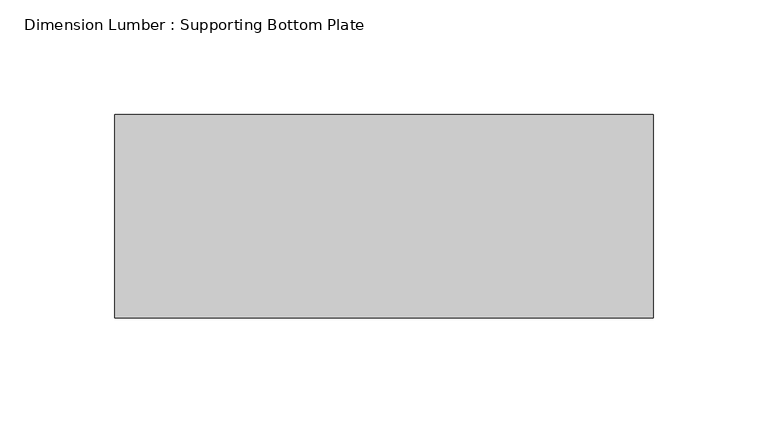
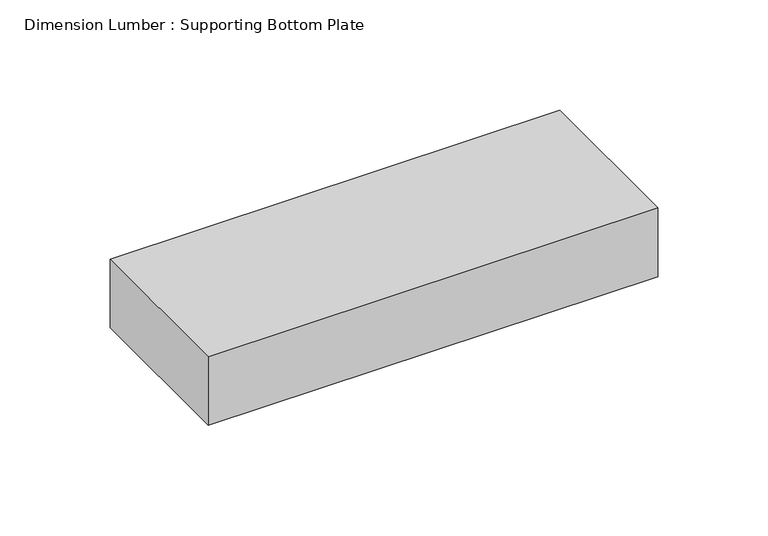
"""IFC4 building model written with IfcOpenShell, lengths in millimetres: beam geometry, Dimension Lumber : Supporting Bottom Plate."""

from ifc_helpers import new_model, si_unit, frame, origin, place, context, project, spatial, polyline, outline, extrude, source, transform, mapped, element, save


def dimension_lumber_supporting_bottom_plate_736f332d(model_context):
    return source(origin(), model_context, "Body", "SweptSolid", [
        extrude(outline(polyline([(139.7000003, 44.45), (139.7000003, -44.45), (-95.2500003, -44.45), (-95.2500003, 44.45), (139.7000003, 44.45)])), frame((0.0, 0.0, -19.05), z_axis=(0.0, 0.0, 1.0), x_axis=(1.0, 0.0, 0.0)), (0.0, 0.0, 1.0), 38.1),
    ])


if __name__ == "__main__":
    model = new_model("IFC4")
    model_context = context("Model", 3, world=origin())
    ifc_project = project(units=[si_unit("LENGTHUNIT", "METRE", prefix="MILLI")], contexts=[model_context])
    site = spatial("IfcSite", under=ifc_project)
    building = spatial("IfcBuilding", under=site)
    placement = place(None, origin())
    dimension_lumber_supporting_bottom_plate_shape = dimension_lumber_supporting_bottom_plate_736f332d(model_context)
    element("IfcBeam", 1, ObjectType="Dimension Lumber : Supporting Bottom Plate", at=placement, inside=building, context=model_context, shape_type="MappedRepresentation", body=[
        mapped(dimension_lumber_supporting_bottom_plate_shape, transform((0.0, 0.0, 0.0), x_axis=(1.0, 0.0, 0.0), y_axis=(0.0, 1.0, 0.0), z_axis=(0.0, 0.0, 1.0))),
    ])
    save(model, "model.ifc")

# Revit data of these elements
# Type "Dimension Lumber : Supporting Bottom Plate"
#   Assembly Code = "B10"
#   A = 0.0364583 SF
#   Length [instance default] = 5' - 0"
#   b = 0' - 3 1/2"
#   d = 0' - 1 1/2"
#   Structural Material [instance default] = Softwood, Lumber
# Element 1 (IfcBeam, "Dimension Lumber : Supporting Bottom Plate")
#   Structural Material = Douglas Fir #2
#   Materials on its faces: "Douglas Fir #2"
# Materials
#   "Softwood, Lumber": class "Wood", colour RGB 223 192 134, transparency 0, Description = "Pinus Echinata", Cost = 0
#   "Douglas Fir #2": class "Wood", colour RGB 223 192 134, transparency 0, Description = "Pinus Echinata", Cost = 0
